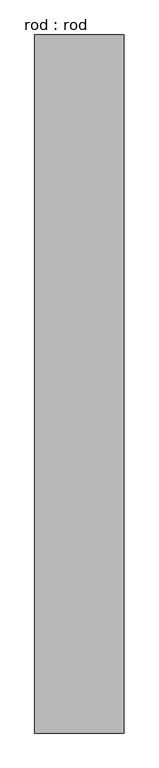
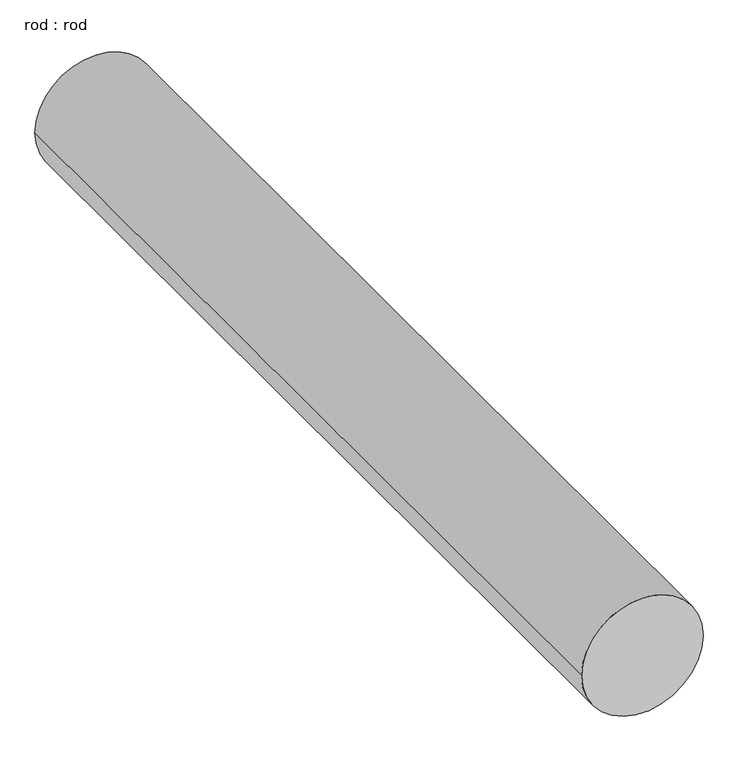
"""IFC4 building model written with IfcOpenShell, lengths in millimetres: proxy geometry, rod : rod."""

from ifc_helpers import new_model, si_unit, point, frame, frame_2d, origin, place, context, project, spatial, circle_curve, trimmed, segment, composite_curve, outline, extrude, source, transform, mapped, element, save


def rod_rod_a097c62b(model_context):
    return source(origin(), model_context, "Body", "SweptSolid", [
        extrude(outline(composite_curve([segment(trimmed(circle_curve(frame_2d((0.0108462, 0.0)), 200.0), [point((0.0108462, 200.0))], [point((0.0108462, -200.0))], False, "CARTESIAN"), True, "CONTINUOUS"), segment(trimmed(circle_curve(frame_2d((0.0108462, 0.0)), 200.0), [point((0.0108462, -200.0))], [point((0.0108462, 200.0))], False, "CARTESIAN"), True, "CONTINUOUS")], self_intersect=False)), frame((0.0, 2533.8000439, 0.0), z_axis=(0.0, 1.0, 0.0), x_axis=(0.0, 0.0, 1.0)), (0.0, 0.0, 1.0), 3117.8571429),
    ])


if __name__ == "__main__":
    model = new_model("IFC4")
    model_context = context("Model", 3, world=origin())
    ifc_project = project(units=[si_unit("LENGTHUNIT", "METRE", prefix="MILLI")], contexts=[model_context])
    site = spatial("IfcSite", under=ifc_project)
    building = spatial("IfcBuilding", under=site)
    placement = place(None, origin())
    rod_rod_shape = rod_rod_a097c62b(model_context)
    element("IfcBuildingElementProxy", 1, Name="rod : rod", ObjectType="rod : rod", at=placement, inside=building, context=model_context, shape_type="MappedRepresentation", body=[
        mapped(rod_rod_shape, transform((0.0, 0.0, 0.0), x_axis=(1.0, 0.0, 0.0), y_axis=(0.0, 1.0, 0.0), z_axis=(0.0, 0.0, 1.0))),
    ])
    save(model, "model.ifc")

# Revit data of these elements
# Type "rod : rod"
#   Default Elevation = 0
